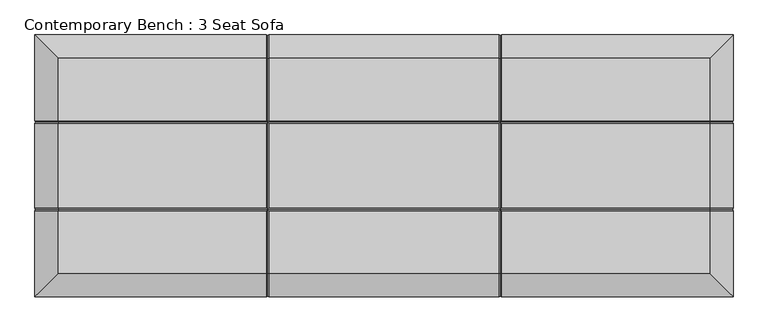
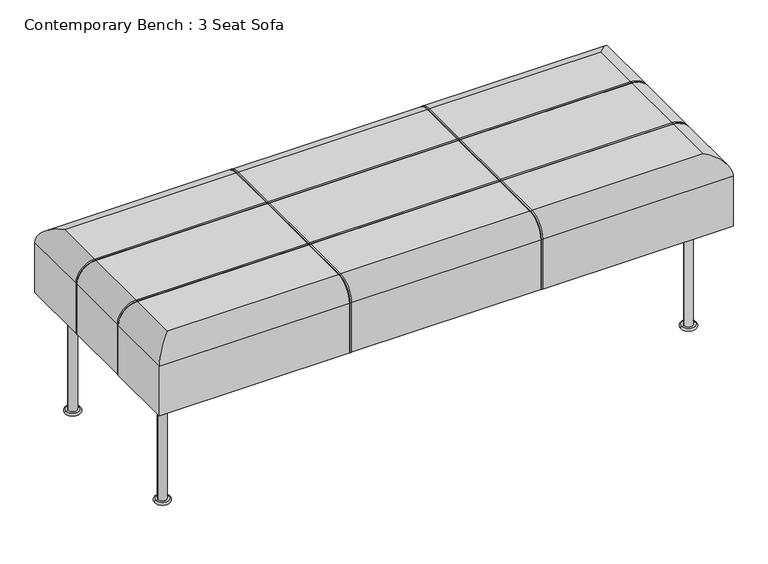
"""IFC4 building model written with IfcOpenShell, lengths in millimetres: furniture geometry, Contemporary Bench : 3 Seat Sofa."""

from ifc_helpers import new_model, si_unit, point, frame, origin, place, context, project, spatial, circle_curve, ellipse_curve, trimmed, source, transform, mapped, element, save
from ifc_brep_helpers import plane_surface, cylinder_surface, revolved_surface, advanced_brep


def contemporary_bench_3_seat_sofa_3fe76763(model_context):
    return source(origin(), model_context, "Body", "AdvancedBrep", [
        advanced_brep(
        [(662.3811933, -50.0, 5.0), (680.3811933, -50.0, 5.0), (680.3811933, -50.0, 250.0), (662.3811933, -50.0, 250.0), (657.3811933, -50.0, 5.0), (685.3811933, -50.0, 5.0), (657.3811933, -50.0, 0.0), (685.3811933, -50.0, 0.0), (671.3811933, -50.0, 0.0), (671.3811933, -50.0, 250.0)],
        [
            (0, 1, circle_curve(frame((671.3811933, -50.0, 5.0), z_axis=(0.0, 0.0, 1.0), x_axis=(1.0, 0.0, 0.0)), 9.0)),
            (1, 2),
            (2, 3, circle_curve(frame((671.3811933, -50.0, 250.0), z_axis=(0.0, 0.0, -1.0), x_axis=(1.0, 0.0, 0.0)), 9.0)),
            (3, 0),
            (1, 0, circle_curve(frame((671.3811933, -50.0, 5.0), z_axis=(0.0, 0.0, 1.0), x_axis=(1.0, 0.0, 0.0)), 9.0)),
            (3, 2, circle_curve(frame((671.3811933, -50.0, 250.0), z_axis=(0.0, 0.0, -1.0), x_axis=(1.0, 0.0, 0.0)), 9.0)),
            (4, 5, circle_curve(frame((671.3811933, -50.0, 5.0), z_axis=(0.0, 0.0, 1.0), x_axis=(1.0, 0.0, 0.0)), 14.0)),
            (5, 1),
            (0, 4),
            (5, 4, circle_curve(frame((671.3811933, -50.0, 5.0), z_axis=(0.0, 0.0, 1.0), x_axis=(1.0, 0.0, 0.0)), 14.0)),
            (6, 7, circle_curve(frame((671.3811933, -50.0, 0.0), z_axis=(0.0, 0.0, 1.0), x_axis=(1.0, 0.0, 0.0)), 14.0)),
            (7, 5, circle_curve(frame((685.3811933, -50.0, 2.5), z_axis=(0.0, -1.0, 0.0), x_axis=(-1.0, 0.0, 0.0)), 2.5)),
            (4, 6, circle_curve(frame((657.3811933, -50.0, 2.5), z_axis=(0.0, -1.0, 0.0), x_axis=(1.0, 0.0, 0.0)), 2.5)),
            (7, 6, circle_curve(frame((671.3811933, -50.0, 0.0), z_axis=(0.0, 0.0, 1.0), x_axis=(1.0, 0.0, 0.0)), 14.0)),
            (8, 7),
            (6, 8),
            (2, 9),
            (9, 3),
        ],
        [
            cylinder_surface(frame((671.3811933, -50.0, -55.0), z_axis=(0.0, 0.0, -1.0), x_axis=(1.0, 0.0, 0.0)), 9.0),
            plane_surface(frame((671.3811933, -50.0, 5.0), z_axis=(0.0, 0.0, 1.0), x_axis=(1.0, 0.0, 0.0))),
            revolved_surface(trimmed(ellipse_curve(frame((685.3811933, -50.0, 2.5), z_axis=(0.0, 1.0, 0.0), x_axis=(-1.0, 0.0, 0.0)), 2.5, 2.5), [point((685.3811933, -50.0, 5.0))], [point((685.3811933, -50.0, 0.0))], True, "CARTESIAN"), (671.3811933, -50.0, -55.0), (0.0, 0.0, -1.0)),
            plane_surface(frame((671.3811933, -50.0, 0.0), z_axis=(0.0, 0.0, -1.0), x_axis=(1.0, 0.0, 0.0))),
            plane_surface(frame((671.3811933, -50.0, 250.0), z_axis=(0.0, 0.0, 1.0), x_axis=(1.0, 0.0, 0.0))),
        ],
        [
            (0, [[1, 2, 3, 4]]),
            (0, [[5, -4, 6, -2]]),
            (1, [[7, 8, -1, 9]]),
            (1, [[10, -9, -5, -8]]),
            (2, [[11, 12, -7, 13]]),
            (2, [[14, -13, -10, -12]]),
            (3, [[15, -11, 16]]),
            (3, [[-16, -14, -15]]),
            (4, [[-3, 17, 18]]),
            (4, [[-6, -18, -17]]),
        ],
    ),
        advanced_brep(
        [(-428.6188067, -50.0, 250.0), (-437.6188067, -50.0, 250.0), (-419.6188067, -50.0, 250.0), (-414.6188067, -50.0, 0.0), (-442.6188067, -50.0, 0.0), (-428.6188067, -50.0, 0.0), (-414.6188067, -50.0, 5.0), (-442.6188067, -50.0, 5.0), (-419.6188067, -50.0, 5.0), (-437.6188067, -50.0, 5.0)],
        [
            (0, 1),
            (1, 2, circle_curve(frame((-428.6188067, -50.0, 250.0), z_axis=(0.0, 0.0, 1.0), x_axis=(-1.0, 0.0, 0.0)), 9.0)),
            (2, 0),
            (2, 1, circle_curve(frame((-428.6188067, -50.0, 250.0), z_axis=(0.0, 0.0, 1.0), x_axis=(-1.0, 0.0, 0.0)), 9.0)),
            (3, 4, circle_curve(frame((-428.6188067, -50.0, 0.0), z_axis=(0.0, 0.0, -1.0), x_axis=(-1.0, 0.0, 0.0)), 14.0)),
            (4, 5),
            (5, 3),
            (4, 3, circle_curve(frame((-428.6188067, -50.0, 0.0), z_axis=(0.0, 0.0, -1.0), x_axis=(-1.0, 0.0, 0.0)), 14.0)),
            (6, 7, circle_curve(frame((-428.6188067, -50.0, 5.0), z_axis=(0.0, 0.0, -1.0), x_axis=(-1.0, 0.0, 0.0)), 14.0)),
            (7, 4, circle_curve(frame((-442.6188067, -50.0, 2.5), z_axis=(0.0, -1.0, 0.0), x_axis=(-1.0, 0.0, 0.0)), 2.5)),
            (3, 6, circle_curve(frame((-414.6188067, -50.0, 2.5), z_axis=(0.0, -1.0, 0.0), x_axis=(1.0, 0.0, 0.0)), 2.5)),
            (7, 6, circle_curve(frame((-428.6188067, -50.0, 5.0), z_axis=(0.0, 0.0, -1.0), x_axis=(-1.0, 0.0, 0.0)), 14.0)),
            (8, 9, circle_curve(frame((-428.6188067, -50.0, 5.0), z_axis=(0.0, 0.0, -1.0), x_axis=(-1.0, 0.0, 0.0)), 9.0)),
            (9, 7),
            (6, 8),
            (9, 8, circle_curve(frame((-428.6188067, -50.0, 5.0), z_axis=(0.0, 0.0, -1.0), x_axis=(-1.0, 0.0, 0.0)), 9.0)),
            (1, 9),
            (8, 2),
        ],
        [
            plane_surface(frame((-428.6188067, -50.0, 250.0), z_axis=(0.0, 0.0, 1.0), x_axis=(-1.0, 0.0, 0.0))),
            plane_surface(frame((-428.6188067, -50.0, 0.0), z_axis=(0.0, 0.0, -1.0), x_axis=(-1.0, 0.0, 0.0))),
            revolved_surface(trimmed(ellipse_curve(frame((-442.6188067, -50.0, 2.5), z_axis=(0.0, 1.0, 0.0), x_axis=(-1.0, 0.0, 0.0)), 2.5, 2.5), [point((-442.6188067, -50.0, 0.0))], [point((-442.6188067, -50.0, 5.0))], True, "CARTESIAN"), (-428.6188067, -50.0, -55.0), (0.0, 0.0, 1.0)),
            plane_surface(frame((-428.6188067, -50.0, 5.0), z_axis=(0.0, 0.0, 1.0), x_axis=(-1.0, 0.0, 0.0))),
            cylinder_surface(frame((-428.6188067, -50.0, -55.0), z_axis=(0.0, 0.0, 1.0), x_axis=(-1.0, 0.0, 0.0)), 9.0),
        ],
        [
            (0, [[1, 2, 3]]),
            (0, [[-3, 4, -1]]),
            (1, [[5, 6, 7]]),
            (1, [[8, -7, -6]]),
            (2, [[9, 10, -5, 11]]),
            (2, [[12, -11, -8, -10]]),
            (3, [[13, 14, -9, 15]]),
            (3, [[16, -15, -12, -14]]),
            (4, [[-2, 17, -13, 18]]),
            (4, [[-4, -18, -16, -17]]),
        ],
    ),
        advanced_brep(
        [(662.3811933, -375.0, 5.0), (680.3811933, -375.0, 5.0), (680.3811933, -375.0, 250.0), (662.3811933, -375.0, 250.0), (657.3811933, -375.0, 5.0), (685.3811933, -375.0, 5.0), (657.3811933, -375.0, 0.0), (685.3811933, -375.0, 0.0), (671.3811933, -375.0, 0.0), (671.3811933, -375.0, 250.0)],
        [
            (0, 1, circle_curve(frame((671.3811933, -375.0, 5.0), z_axis=(0.0, 0.0, 1.0), x_axis=(0.9999999999999999, 0.0, 0.0)), 9.0)),
            (1, 2),
            (2, 3, circle_curve(frame((671.3811933, -375.0, 250.0), z_axis=(0.0, 0.0, -1.0), x_axis=(0.9999999999999999, 0.0, 0.0)), 9.0)),
            (3, 0),
            (1, 0, circle_curve(frame((671.3811933, -375.0, 5.0), z_axis=(0.0, 0.0, 1.0), x_axis=(0.9999999999999999, 0.0, 0.0)), 9.0)),
            (3, 2, circle_curve(frame((671.3811933, -375.0, 250.0), z_axis=(0.0, 0.0, -1.0), x_axis=(0.9999999999999999, 0.0, 0.0)), 9.0)),
            (4, 5, circle_curve(frame((671.3811933, -375.0, 5.0), z_axis=(0.0, 0.0, 1.0), x_axis=(0.9999999999999999, 0.0, 0.0)), 14.0)),
            (5, 1),
            (0, 4),
            (5, 4, circle_curve(frame((671.3811933, -375.0, 5.0), z_axis=(0.0, 0.0, 1.0), x_axis=(0.9999999999999999, 0.0, 0.0)), 14.0)),
            (6, 7, circle_curve(frame((671.3811933, -375.0, 0.0), z_axis=(0.0, 0.0, 1.0), x_axis=(0.9999999999999999, 0.0, 0.0)), 14.0)),
            (7, 5, circle_curve(frame((685.3811933, -375.0, 2.5), z_axis=(0.0, -1.0, 0.0), x_axis=(0.9999999999999999, 0.0, 0.0)), 2.5)),
            (4, 6, circle_curve(frame((657.3811933, -375.0, 2.5), z_axis=(0.0, -1.0, 0.0), x_axis=(-0.9999999999999999, 0.0, 0.0)), 2.5)),
            (7, 6, circle_curve(frame((671.3811933, -375.0, 0.0), z_axis=(0.0, 0.0, 1.0), x_axis=(0.9999999999999999, 0.0, 0.0)), 14.0)),
            (8, 7),
            (6, 8),
            (2, 9),
            (9, 3),
        ],
        [
            cylinder_surface(frame((671.3811933, -375.0, -55.0), z_axis=(0.0, 0.0, -0.9999999999999999), x_axis=(0.9999999999999999, 0.0, 0.0)), 9.0),
            plane_surface(frame((671.3811933, -375.0, 5.0), z_axis=(0.0, 0.0, 1.0), x_axis=(1.0, 0.0, 0.0))),
            revolved_surface(trimmed(ellipse_curve(frame((685.3811933, -375.0, 2.5), z_axis=(0.0, 1.0, 0.0), x_axis=(0.9999999999999999, 0.0, 0.0)), 2.5, 2.5), [point((685.3811933, -375.0, 5.0))], [point((685.3811933, -375.0, 0.0))], True, "CARTESIAN"), (671.3811933, -375.0, -55.0), (0.0, 0.0, -0.9999999999999999)),
            plane_surface(frame((671.3811933, -375.0, 0.0), z_axis=(0.0, 0.0, -1.0), x_axis=(1.0, 0.0, 0.0))),
            plane_surface(frame((671.3811933, -375.0, 250.0), z_axis=(0.0, 0.0, 1.0), x_axis=(1.0, 0.0, 0.0))),
        ],
        [
            (0, [[1, 2, 3, 4]]),
            (0, [[5, -4, 6, -2]]),
            (1, [[7, 8, -1, 9]]),
            (1, [[10, -9, -5, -8]]),
            (2, [[11, 12, -7, 13]]),
            (2, [[14, -13, -10, -12]]),
            (3, [[15, -11, 16]]),
            (3, [[-16, -14, -15]]),
            (4, [[-3, 17, 18]]),
            (4, [[-6, -18, -17]]),
        ],
    ),
        advanced_brep(
        [(-428.6188067, -375.0, 250.0), (-437.6188067, -375.0, 250.0), (-419.6188067, -375.0, 250.0), (-414.6188067, -375.0, 0.0), (-442.6188067, -375.0, 0.0), (-428.6188067, -375.0, 0.0), (-414.6188067, -375.0, 5.0), (-442.6188067, -375.0, 5.0), (-419.6188067, -375.0, 5.0), (-437.6188067, -375.0, 5.0)],
        [
            (0, 1),
            (1, 2, circle_curve(frame((-428.6188067, -375.0, 250.0), z_axis=(0.0, 0.0, 1.0), x_axis=(-1.0, 0.0, 0.0)), 9.0)),
            (2, 0),
            (2, 1, circle_curve(frame((-428.6188067, -375.0, 250.0), z_axis=(0.0, 0.0, 1.0), x_axis=(-1.0, 0.0, 0.0)), 9.0)),
            (3, 4, circle_curve(frame((-428.6188067, -375.0, 0.0), z_axis=(0.0, 0.0, -1.0), x_axis=(-1.0, 0.0, 0.0)), 14.0)),
            (4, 5),
            (5, 3),
            (4, 3, circle_curve(frame((-428.6188067, -375.0, 0.0), z_axis=(0.0, 0.0, -1.0), x_axis=(-1.0, 0.0, 0.0)), 14.0)),
            (6, 7, circle_curve(frame((-428.6188067, -375.0, 5.0), z_axis=(0.0, 0.0, -1.0), x_axis=(-1.0, 0.0, 0.0)), 14.0)),
            (7, 4, circle_curve(frame((-442.6188067, -375.0, 2.5), z_axis=(0.0, -1.0, 0.0), x_axis=(-1.0, 0.0, 0.0)), 2.5)),
            (3, 6, circle_curve(frame((-414.6188067, -375.0, 2.5), z_axis=(0.0, -1.0, 0.0), x_axis=(1.0, 0.0, 0.0)), 2.5)),
            (7, 6, circle_curve(frame((-428.6188067, -375.0, 5.0), z_axis=(0.0, 0.0, -1.0), x_axis=(-1.0, 0.0, 0.0)), 14.0)),
            (8, 9, circle_curve(frame((-428.6188067, -375.0, 5.0), z_axis=(0.0, 0.0, -1.0), x_axis=(-1.0, 0.0, 0.0)), 9.0)),
            (9, 7),
            (6, 8),
            (9, 8, circle_curve(frame((-428.6188067, -375.0, 5.0), z_axis=(0.0, 0.0, -1.0), x_axis=(-1.0, 0.0, 0.0)), 9.0)),
            (1, 9),
            (8, 2),
        ],
        [
            plane_surface(frame((-428.6188067, -375.0, 250.0), z_axis=(0.0, 0.0, 1.0), x_axis=(-1.0, 0.0, 0.0))),
            plane_surface(frame((-428.6188067, -375.0, 0.0), z_axis=(0.0, 0.0, -1.0), x_axis=(-1.0, 0.0, 0.0))),
            revolved_surface(trimmed(ellipse_curve(frame((-442.6188067, -375.0, 2.5), z_axis=(0.0, 1.0, 0.0), x_axis=(-1.0, 0.0, 0.0)), 2.5, 2.5), [point((-442.6188067, -375.0, 0.0))], [point((-442.6188067, -375.0, 5.0))], True, "CARTESIAN"), (-428.6188067, -375.0, -55.0), (0.0, 0.0, 1.0)),
            plane_surface(frame((-428.6188067, -375.0, 5.0), z_axis=(0.0, 0.0, 1.0), x_axis=(-1.0, 0.0, 0.0))),
            cylinder_surface(frame((-428.6188067, -375.0, -55.0), z_axis=(0.0, 0.0, 1.0), x_axis=(-1.0, 0.0, 0.0)), 9.0),
        ],
        [
            (0, [[1, 2, 3]]),
            (0, [[-3, 4, -1]]),
            (1, [[5, 6, 7]]),
            (1, [[8, -7, -6]]),
            (2, [[9, 10, -5, 11]]),
            (2, [[12, -11, -8, -10]]),
            (3, [[13, 14, -9, 15]]),
            (3, [[16, -15, -12, -14]]),
            (4, [[-2, 17, -13, 18]]),
            (4, [[-4, -18, -16, -17]]),
        ],
    ),
        advanced_brep(
        [(-478.6188067, -450.0, 360.0), (-478.6188067, -450.0, 250.0), (-81.2982159, -450.0, 250.0), (-81.2982159, -450.0, 360.0), (721.3811933, -450.0, 250.0), (721.3811933, -450.0, 360.0), (324.0606025, -450.0, 360.0), (324.0606025, -450.0, 250.0), (-75.9393975, -450.0, 250.0), (318.7017841, -450.0, 250.0), (318.7017841, -450.0, 360.0), (-75.9393975, -450.0, 360.0), (721.3811933, 0.0, 360.0), (721.3811933, 0.0, 250.0), (324.0606025, 0.0, 250.0), (324.0606025, 0.0, 360.0), (-478.6188067, 0.0, 250.0), (-478.6188067, 0.0, 360.0), (-81.2982159, 0.0, 360.0), (-81.2982159, 0.0, 250.0), (318.7017841, 0.0, 250.0), (-75.9393975, 0.0, 250.0), (-75.9393975, 0.0, 360.0), (318.7017841, 0.0, 360.0), (-438.6188067, -302.679408, 400.0), (-438.6188067, -410.0, 400.0), (-81.2982159, -410.0, 400.0), (-81.2982159, -302.6794092, 400.0), (-438.6188067, -40.0, 400.0), (-438.6188067, -147.3205908, 400.0), (-81.2982159, -147.3205908, 400.0), (-81.2982159, -40.0, 400.0), (-438.6188067, -152.6794084, 400.0), (-438.6188067, -297.3205908, 400.0), (-81.2982159, -297.3205908, 400.0), (-81.2982159, -152.6794092, 400.0), (681.3811933, -410.0, 400.0), (681.3811933, -302.6794092, 400.0), (324.0606025, -302.6794092, 400.0), (324.0606025, -410.0, 400.0), (681.3811933, -147.3205908, 400.0), (681.3811933, -40.0, 400.0), (324.0606025, -40.0, 400.0), (324.0606025, -147.3205908, 400.0), (681.3811933, -297.3205908, 400.0), (681.3811933, -152.6794092, 400.0), (324.0606025, -152.6794092, 400.0), (324.0606025, -297.3205908, 400.0), (318.7017854, -40.0, 400.0), (-75.9393975, -40.0, 400.0), (-75.9393975, -147.3205908, 400.0), (318.7017841, -147.3205908, 400.0), (-75.9393975, -410.0, 400.0), (318.7017841, -410.0, 400.0), (318.7017841, -302.6794092, 400.0), (-75.9393975, -302.6794092, 400.0), (-75.9393975, -297.3205908, 400.0), (318.7017841, -297.3205908, 400.0), (318.7017841, -152.6794092, 400.0), (-75.9393975, -152.6794092, 400.0), (-478.6188067, -302.6794092, 360.0), (-478.6188067, -302.6794092, 250.0), (-478.6188067, -147.3205908, 250.0), (-478.6188067, -147.3205908, 360.0), (-478.6188067, -297.3205908, 360.0), (-478.6188067, -152.6794092, 360.0), (-478.6188067, -152.6794092, 250.0), (-478.6188067, -297.3205908, 250.0), (-475.9393975, -300.0, 250.0), (-475.9393975, -150.0, 250.0), (-78.6188067, -2.6794092, 250.0), (321.3811933, -2.6794092, 250.0), (721.3811933, -147.3205908, 250.0), (718.7017841, -150.0, 250.0), (721.3811933, -152.6794092, 250.0), (721.3811933, -297.3205908, 250.0), (718.7017841, -300.0, 250.0), (721.3811933, -302.6794092, 250.0), (321.3811933, -447.3205908, 250.0), (-78.6188067, -447.3205908, 250.0), (721.3811933, -302.6794092, 360.0), (721.3811933, -147.3205908, 360.0), (721.3811933, -152.6794092, 360.0), (721.3811933, -297.3205908, 360.0), (-475.9393975, -300.0, 360.0), (-475.9393975, -150.0, 360.0), (-438.6188067, -300.0, 397.3205908), (-438.6188067, -150.0, 397.3205908), (-78.6188067, -300.0, 397.3205908), (321.3811933, -300.0, 397.3205908), (681.3811933, -300.0, 397.3205908), (-78.6188067, -150.0, 397.3205908), (321.3811933, -150.0, 397.3205908), (681.3811933, -150.0, 397.3205908), (718.7017841, -300.0, 360.0), (718.7017841, -150.0, 360.0), (-78.6188067, -2.6794092, 360.0), (321.3811933, -2.6794092, 360.0), (-78.6188067, -40.0, 397.3205908), (321.3811933, -40.0, 397.3205908), (-78.6188067, -410.0, 397.3205908), (321.3811933, -410.0, 397.3205908), (-78.6188067, -447.3205908, 360.0), (321.3811933, -447.3205908, 360.0)],
        [
            (0, 1),
            (1, 2),
            (2, 3),
            (3, 0),
            (4, 5),
            (5, 6),
            (6, 7),
            (7, 4),
            (8, 9),
            (9, 10),
            (10, 11),
            (11, 8),
            (12, 13),
            (13, 14),
            (14, 15),
            (15, 12),
            (16, 17),
            (17, 18),
            (18, 19),
            (19, 16),
            (20, 21),
            (21, 22),
            (22, 23),
            (23, 20),
            (24, 25),
            (25, 26),
            (26, 27),
            (27, 24),
            (28, 29),
            (29, 30),
            (30, 31),
            (31, 28),
            (32, 33),
            (33, 34),
            (34, 35),
            (35, 32),
            (36, 37),
            (37, 38),
            (38, 39),
            (39, 36),
            (40, 41),
            (41, 42),
            (42, 43),
            (43, 40),
            (44, 45),
            (45, 46),
            (46, 47),
            (47, 44),
            (48, 49),
            (49, 50),
            (50, 51),
            (51, 48),
            (52, 53),
            (53, 54),
            (54, 55),
            (55, 52),
            (56, 57),
            (57, 58),
            (58, 59),
            (59, 56),
            (0, 60),
            (60, 61),
            (61, 1),
            (16, 62),
            (62, 63),
            (63, 17),
            (64, 65),
            (65, 66),
            (66, 67),
            (67, 64),
            (61, 68, circle_curve(frame((-475.9393975, -302.6794092, 250.0), z_axis=(0.0, 0.0, -1.0), x_axis=(1.0, 0.0, 0.0)), 2.6794092)),
            (68, 67, circle_curve(frame((-475.9393975, -297.3205908, 250.0), z_axis=(0.0, 0.0, -1.0), x_axis=(1.0, 0.0, 0.0)), 2.6794092)),
            (66, 69, circle_curve(frame((-475.9393975, -152.6794092, 250.0), z_axis=(0.0, 0.0, -1.0), x_axis=(1.0, 0.0, 0.0)), 2.6794092)),
            (69, 62, circle_curve(frame((-475.9393975, -147.3205908, 250.0), z_axis=(0.0, 0.0, -1.0), x_axis=(1.0, 0.0, 0.0)), 2.6794092)),
            (19, 70, circle_curve(frame((-81.2982159, -2.6794092, 250.0), z_axis=(0.0, 0.0, -1.0), x_axis=(1.0, 0.0, 0.0)), 2.6794092)),
            (70, 21, circle_curve(frame((-75.9393975, -2.6794092, 250.0), z_axis=(0.0, 0.0, -1.0), x_axis=(1.0, 0.0, 0.0)), 2.6794092)),
            (20, 71, circle_curve(frame((318.7017841, -2.6794092, 250.0), z_axis=(0.0, 0.0, -1.0), x_axis=(1.0, 0.0, 0.0)), 2.6794092)),
            (71, 14, circle_curve(frame((324.0606025, -2.6794092, 250.0), z_axis=(0.0, 0.0, -1.0), x_axis=(1.0, 0.0, 0.0)), 2.6794092)),
            (13, 72),
            (72, 73, circle_curve(frame((718.7017841, -147.3205908, 250.0), z_axis=(0.0, 0.0, -1.0), x_axis=(-1.0, 0.0, 0.0)), 2.6794092)),
            (73, 74, circle_curve(frame((718.7017841, -152.6794092, 250.0), z_axis=(0.0, 0.0, -1.0), x_axis=(-1.0, 0.0, 0.0)), 2.6794092)),
            (74, 75),
            (75, 76, circle_curve(frame((718.7017841, -297.3205908, 250.0), z_axis=(0.0, 0.0, -1.0), x_axis=(-1.0, 0.0, 0.0)), 2.6794092)),
            (76, 77, circle_curve(frame((718.7017841, -302.6794092, 250.0), z_axis=(0.0, 0.0, -1.0), x_axis=(-1.0, 0.0, 0.0)), 2.6794092)),
            (77, 4),
            (7, 78, circle_curve(frame((324.0606025, -447.3205908, 250.0), z_axis=(0.0, 0.0, -1.0), x_axis=(1.0, 0.0, 0.0)), 2.6794092)),
            (78, 9, circle_curve(frame((318.7017841, -447.3205908, 250.0), z_axis=(0.0, 0.0, -1.0), x_axis=(1.0, 0.0, 0.0)), 2.6794092)),
            (8, 79, circle_curve(frame((-75.9393975, -447.3205908, 250.0), z_axis=(0.0, 0.0, -1.0), x_axis=(1.0, 0.0, 0.0)), 2.6794092)),
            (79, 2, circle_curve(frame((-81.2982159, -447.3205908, 250.0), z_axis=(0.0, 0.0, -1.0), x_axis=(1.0, 0.0, 0.0)), 2.6794092)),
            (77, 80),
            (80, 5),
            (12, 81),
            (81, 72),
            (74, 82),
            (82, 83),
            (83, 75),
            (32, 65, circle_curve(frame((-438.6188067, -152.6794092, 360.0), z_axis=(0.0, -1.0, 0.0), x_axis=(-1.0, 0.0, 0.0)), 40.0)),
            (64, 33, circle_curve(frame((-438.6188067, -297.3205908, 360.0), z_axis=(0.0, 1.0, 0.0), x_axis=(-1.0, 0.0, 0.0)), 40.0)),
            (28, 17, ellipse_curve(frame((-438.6188067, -40.0, 360.0), z_axis=(-0.7071067811865475, -0.7071067811865475, 0.0), x_axis=(-0.7071067811865474, 0.7071067811865476, 0.0)), 56.5685425, 40.0)),
            (63, 29, circle_curve(frame((-438.6188067, -147.3205908, 360.0), z_axis=(0.0, 1.0, 0.0), x_axis=(-1.0, 0.0, 0.0)), 40.0)),
            (0, 25, ellipse_curve(frame((-438.6188067, -410.0, 360.0), z_axis=(-0.7071067811865475, 0.7071067811865475, 0.0), x_axis=(0.7071067811865474, 0.7071067811865476, 0.0)), 56.5685425, 40.0)),
            (24, 60, circle_curve(frame((-438.6188067, -302.6794092, 360.0), z_axis=(0.0, -1.0, 0.0), x_axis=(-1.0, 0.0, 0.0)), 40.0)),
            (22, 49, circle_curve(frame((-75.9393975, -40.0, 360.0), z_axis=(1.0, 0.0, 0.0), x_axis=(0.0, 1.0, 0.0)), 40.0)),
            (48, 23, circle_curve(frame((318.7017841, -40.0, 360.0), z_axis=(-1.0, 0.0, 0.0), x_axis=(0.0, 1.0, 0.0)), 40.0)),
            (31, 18, circle_curve(frame((-81.2982159, -40.0, 360.0), z_axis=(-1.0, 0.0, 0.0), x_axis=(0.0, 1.0, 0.0)), 40.0)),
            (41, 12, ellipse_curve(frame((681.3811933, -40.0, 360.0), z_axis=(-0.7071067811865475, 0.7071067811865475, 0.0), x_axis=(0.7071067811865476, 0.7071067811865474, 0.0)), 56.5685425, 40.0)),
            (15, 42, circle_curve(frame((324.0606025, -40.0, 360.0), z_axis=(1.0, 0.0, 0.0), x_axis=(0.0, 1.0, 0.0)), 40.0)),
            (44, 83, circle_curve(frame((681.3811933, -297.3205908, 360.0), z_axis=(0.0, 1.0, 0.0), x_axis=(1.0, 0.0, 0.0)), 40.0)),
            (82, 45, circle_curve(frame((681.3811933, -152.6794092, 360.0), z_axis=(0.0, -1.0, 0.0), x_axis=(1.0, 0.0, 0.0)), 40.0)),
            (40, 81, circle_curve(frame((681.3811933, -147.3205908, 360.0), z_axis=(0.0, 1.0, 0.0), x_axis=(1.0, 0.0, 0.0)), 40.0)),
            (36, 5, ellipse_curve(frame((681.3811933, -410.0, 360.0), z_axis=(0.7071067811865475, 0.7071067811865475, 0.0), x_axis=(0.7071067811865474, -0.7071067811865476, 0.0)), 56.5685425, 40.0)),
            (80, 37, circle_curve(frame((681.3811933, -302.6794092, 360.0), z_axis=(0.0, -1.0, 0.0), x_axis=(1.0, 0.0, 0.0)), 40.0)),
            (10, 53, circle_curve(frame((318.7017841, -410.0, 360.0), z_axis=(-1.0, 0.0, 0.0), x_axis=(0.0, -1.0, 0.0)), 40.0)),
            (52, 11, circle_curve(frame((-75.9393975, -410.0, 360.0), z_axis=(1.0, 0.0, 0.0), x_axis=(0.0, -1.0, 0.0)), 40.0)),
            (3, 26, circle_curve(frame((-81.2982159, -410.0, 360.0), z_axis=(-1.0, 0.0, 0.0), x_axis=(0.0, -1.0, 0.0)), 40.0)),
            (39, 6, circle_curve(frame((324.0606025, -410.0, 360.0), z_axis=(1.0, 0.0, 0.0), x_axis=(0.0, -1.0, 0.0)), 40.0)),
            (68, 84),
            (84, 64, circle_curve(frame((-475.9393975, -297.3205908, 360.0), z_axis=(0.0, 0.0, -1.0), x_axis=(1.0, 0.0, 0.0)), 2.6794092)),
            (60, 84, circle_curve(frame((-475.9393975, -302.6794092, 360.0), z_axis=(0.0, 0.0, -1.0), x_axis=(1.0, 0.0, 0.0)), 2.6794092)),
            (69, 85),
            (85, 63, circle_curve(frame((-475.9393975, -147.3205908, 360.0), z_axis=(0.0, 0.0, -1.0), x_axis=(1.0, 0.0, 0.0)), 2.6794092)),
            (65, 85, circle_curve(frame((-475.9393975, -152.6794092, 360.0), z_axis=(0.0, 0.0, -1.0), x_axis=(1.0, 0.0, 0.0)), 2.6794092)),
            (84, 86, circle_curve(frame((-438.6188067, -300.0, 360.0), z_axis=(0.0, 1.0, 0.0), x_axis=(-1.0, 0.0, 0.0)), 37.3205908)),
            (86, 33, circle_curve(frame((-438.6188067, -297.3205908, 397.3205908), z_axis=(-1.0, 0.0, 0.0), x_axis=(0.0, 0.0, -1.0)), 2.6794092)),
            (24, 86, circle_curve(frame((-438.6188067, -302.6794092, 397.3205908), z_axis=(-1.0, 0.0, 0.0), x_axis=(0.0, 0.0, -1.0)), 2.6794092)),
            (85, 87, circle_curve(frame((-438.6188067, -150.0, 360.0), z_axis=(0.0, 1.0, 0.0), x_axis=(-1.0, 0.0, 0.0)), 37.3205908)),
            (87, 29, circle_curve(frame((-438.6188067, -147.3205908, 397.3205908), z_axis=(-1.0, 0.0, 0.0), x_axis=(0.0, 0.0, -1.0)), 2.6794092)),
            (32, 87, circle_curve(frame((-438.6188067, -152.6794092, 397.3205908), z_axis=(-1.0, 0.0, 0.0), x_axis=(0.0, 0.0, -1.0)), 2.6794092)),
            (56, 88, ellipse_curve(frame((-75.9393975, -297.3205908, 397.3205908), z_axis=(0.7071067811865464, -0.7071067811865487, 0.0), x_axis=(0.7071067811865487, 0.7071067811865464, 0.0)), 3.7892569, 2.6794092)),
            (88, 89),
            (89, 57, ellipse_curve(frame((318.7017841, -297.3205908, 397.3205908), z_axis=(-0.7071067811865487, -0.7071067811865464, 0.0), x_axis=(0.7071067811865465, -0.7071067811865487, 0.0)), 3.7892569, 2.6794092)),
            (86, 88),
            (88, 34, ellipse_curve(frame((-81.2982159, -297.3205908, 397.3205908), z_axis=(-0.7071067811865487, -0.7071067811865464, 0.0), x_axis=(0.7071067811865465, -0.7071067811865487, 0.0)), 3.7892569, 2.6794092)),
            (90, 44, circle_curve(frame((681.3811933, -297.3205908, 397.3205908), z_axis=(-1.0, 0.0, 0.0), x_axis=(0.0, 0.0, -1.0)), 2.6794092)),
            (47, 89, ellipse_curve(frame((324.0606025, -297.3205908, 397.3205908), z_axis=(0.7071067811865464, -0.7071067811865487, 0.0), x_axis=(0.7071067811865487, 0.7071067811865464, 0.0)), 3.7892569, 2.6794092)),
            (89, 90),
            (54, 89, ellipse_curve(frame((318.7017841, -302.6794092, 397.3205908), z_axis=(-0.7071067811865464, 0.7071067811865487, 0.0), x_axis=(0.7071067811865487, 0.7071067811865464, 0.0)), 3.7892569, 2.6794092)),
            (88, 55, ellipse_curve(frame((-75.9393975, -302.6794092, 397.3205908), z_axis=(0.7071067811865487, 0.7071067811865464, 0.0), x_axis=(0.7071067811865465, -0.7071067811865487, 0.0)), 3.7892569, 2.6794092)),
            (27, 88, ellipse_curve(frame((-81.2982159, -302.6794092, 397.3205908), z_axis=(-0.7071067811865464, 0.7071067811865487, 0.0), x_axis=(0.7071067811865487, 0.7071067811865464, 0.0)), 3.7892569, 2.6794092)),
            (37, 90, circle_curve(frame((681.3811933, -302.6794092, 397.3205908), z_axis=(-1.0, 0.0, 0.0), x_axis=(0.0, 0.0, -1.0)), 2.6794092)),
            (89, 38, ellipse_curve(frame((324.0606025, -302.6794092, 397.3205908), z_axis=(0.7071067811865487, 0.7071067811865464, 0.0), x_axis=(0.7071067811865465, -0.7071067811865487, 0.0)), 3.7892569, 2.6794092)),
            (50, 91, ellipse_curve(frame((-75.9393975, -147.3205908, 397.3205908), z_axis=(0.7071067811865464, -0.7071067811865487, 0.0), x_axis=(0.7071067811865487, 0.7071067811865464, 0.0)), 3.7892569, 2.6794092)),
            (91, 92),
            (92, 51, ellipse_curve(frame((318.7017841, -147.3205908, 397.3205908), z_axis=(-0.7071067811865487, -0.7071067811865464, 0.0), x_axis=(0.7071067811865465, -0.7071067811865487, 0.0)), 3.7892569, 2.6794092)),
            (87, 91),
            (91, 30, ellipse_curve(frame((-81.2982159, -147.3205908, 397.3205908), z_axis=(-0.7071067811865487, -0.7071067811865464, 0.0), x_axis=(0.7071067811865465, -0.7071067811865487, 0.0)), 3.7892569, 2.6794092)),
            (93, 40, circle_curve(frame((681.3811933, -147.3205908, 397.3205908), z_axis=(-1.0, 0.0, 0.0), x_axis=(0.0, 0.0, -1.0)), 2.6794092)),
            (43, 92, ellipse_curve(frame((324.0606025, -147.3205908, 397.3205908), z_axis=(0.7071067811865464, -0.7071067811865487, 0.0), x_axis=(0.7071067811865487, 0.7071067811865464, 0.0)), 3.7892569, 2.6794092)),
            (92, 93),
            (58, 92, ellipse_curve(frame((318.7017841, -152.6794092, 397.3205908), z_axis=(-0.7071067811865464, 0.7071067811865487, 0.0), x_axis=(0.7071067811865487, 0.7071067811865464, 0.0)), 3.7892569, 2.6794092)),
            (91, 59, ellipse_curve(frame((-75.9393975, -152.6794092, 397.3205908), z_axis=(0.7071067811865487, 0.7071067811865464, 0.0), x_axis=(0.7071067811865465, -0.7071067811865487, 0.0)), 3.7892569, 2.6794092)),
            (35, 91, ellipse_curve(frame((-81.2982159, -152.6794092, 397.3205908), z_axis=(-0.7071067811865464, 0.7071067811865487, 0.0), x_axis=(0.7071067811865487, 0.7071067811865464, 0.0)), 3.7892569, 2.6794092)),
            (45, 93, circle_curve(frame((681.3811933, -152.6794092, 397.3205908), z_axis=(-1.0, 0.0, 0.0), x_axis=(0.0, 0.0, -1.0)), 2.6794092)),
            (92, 46, ellipse_curve(frame((324.0606025, -152.6794092, 397.3205908), z_axis=(0.7071067811865487, 0.7071067811865464, 0.0), x_axis=(0.7071067811865465, -0.7071067811865487, 0.0)), 3.7892569, 2.6794092)),
            (90, 94, circle_curve(frame((681.3811933, -300.0, 360.0), z_axis=(0.0, 1.0, 0.0), x_axis=(0.0, 0.0, 1.0)), 37.3205908)),
            (94, 83, circle_curve(frame((718.7017841, -297.3205908, 360.0), z_axis=(0.0, 0.0, 1.0), x_axis=(-1.0, 0.0, 0.0)), 2.6794092)),
            (80, 94, circle_curve(frame((718.7017841, -302.6794092, 360.0), z_axis=(0.0, 0.0, 1.0), x_axis=(-1.0, 0.0, 0.0)), 2.6794092)),
            (93, 95, circle_curve(frame((681.3811933, -150.0, 360.0), z_axis=(0.0, 1.0, 0.0), x_axis=(0.0, 0.0, 1.0)), 37.3205908)),
            (95, 81, circle_curve(frame((718.7017841, -147.3205908, 360.0), z_axis=(0.0, 0.0, 1.0), x_axis=(-1.0, 0.0, 0.0)), 2.6794092)),
            (82, 95, circle_curve(frame((718.7017841, -152.6794092, 360.0), z_axis=(0.0, 0.0, 1.0), x_axis=(-1.0, 0.0, 0.0)), 2.6794092)),
            (94, 76),
            (95, 73),
            (70, 96),
            (96, 22, circle_curve(frame((-75.9393975, -2.6794092, 360.0), z_axis=(0.0, 0.0, -1.0), x_axis=(1.0, 0.0, 0.0)), 2.6794092)),
            (18, 96, circle_curve(frame((-81.2982159, -2.6794092, 360.0), z_axis=(0.0, 0.0, -1.0), x_axis=(1.0, 0.0, 0.0)), 2.6794092)),
            (71, 97),
            (97, 15, circle_curve(frame((324.0606025, -2.6794092, 360.0), z_axis=(0.0, 0.0, -1.0), x_axis=(1.0, 0.0, 0.0)), 2.6794092)),
            (23, 97, circle_curve(frame((318.7017841, -2.6794092, 360.0), z_axis=(0.0, 0.0, -1.0), x_axis=(1.0, 0.0, 0.0)), 2.6794092)),
            (96, 98, circle_curve(frame((-78.6188067, -40.0, 360.0), z_axis=(1.0, 0.0, 0.0), x_axis=(0.0, 1.0, 0.0)), 37.3205908)),
            (98, 49, circle_curve(frame((-75.9393975, -40.0, 397.3205908), z_axis=(0.0, 1.0, 0.0), x_axis=(1.0, 0.0, 0.0)), 2.6794092)),
            (31, 98, circle_curve(frame((-81.2982159, -40.0, 397.3205908), z_axis=(0.0, 1.0, 0.0), x_axis=(1.0, 0.0, 0.0)), 2.6794092)),
            (97, 99, circle_curve(frame((321.3811933, -40.0, 360.0), z_axis=(1.0, 0.0, 0.0), x_axis=(0.0, 1.0, 0.0)), 37.3205908)),
            (99, 42, circle_curve(frame((324.0606025, -40.0, 397.3205908), z_axis=(0.0, 1.0, 0.0), x_axis=(1.0, 0.0, 0.0)), 2.6794092)),
            (48, 99, circle_curve(frame((318.7017841, -40.0, 397.3205908), z_axis=(0.0, 1.0, 0.0), x_axis=(1.0, 0.0, 0.0)), 2.6794092)),
            (98, 91),
            (100, 52, circle_curve(frame((-75.9393975, -410.0, 397.3205908), z_axis=(0.0, 1.0, 0.0), x_axis=(1.0, 0.0, 0.0)), 2.6794092)),
            (88, 100),
            (91, 88),
            (26, 100, circle_curve(frame((-81.2982159, -410.0, 397.3205908), z_axis=(0.0, 1.0, 0.0), x_axis=(1.0, 0.0, 0.0)), 2.6794092)),
            (99, 92),
            (101, 39, circle_curve(frame((324.0606025, -410.0, 397.3205908), z_axis=(0.0, 1.0, 0.0), x_axis=(1.0, 0.0, 0.0)), 2.6794092)),
            (89, 101),
            (92, 89),
            (53, 101, circle_curve(frame((318.7017841, -410.0, 397.3205908), z_axis=(0.0, 1.0, 0.0), x_axis=(1.0, 0.0, 0.0)), 2.6794092)),
            (100, 102, circle_curve(frame((-78.6188067, -410.0, 360.0), z_axis=(1.0, 0.0, 0.0), x_axis=(0.0, 0.0, 1.0)), 37.3205908)),
            (102, 11, circle_curve(frame((-75.9393975, -447.3205908, 360.0), z_axis=(0.0, 0.0, 1.0), x_axis=(1.0, 0.0, 0.0)), 2.6794092)),
            (3, 102, circle_curve(frame((-81.2982159, -447.3205908, 360.0), z_axis=(0.0, 0.0, 1.0), x_axis=(1.0, 0.0, 0.0)), 2.6794092)),
            (101, 103, circle_curve(frame((321.3811933, -410.0, 360.0), z_axis=(1.0, 0.0, 0.0), x_axis=(0.0, 0.0, 1.0)), 37.3205908)),
            (103, 6, circle_curve(frame((324.0606025, -447.3205908, 360.0), z_axis=(0.0, 0.0, 1.0), x_axis=(1.0, 0.0, 0.0)), 2.6794092)),
            (10, 103, circle_curve(frame((318.7017841, -447.3205908, 360.0), z_axis=(0.0, 0.0, 1.0), x_axis=(1.0, 0.0, 0.0)), 2.6794092)),
            (102, 79),
            (103, 78),
        ],
        [
            plane_surface(frame((-478.6188067, -450.0, 400.0), z_axis=(0.0, -1.0, 0.0), x_axis=(-1.0, 0.0, 0.0))),
            plane_surface(frame((-478.6188067, 0.0, 400.0), z_axis=(0.0, 1.0, 0.0), x_axis=(1.0, 0.0, 0.0))),
            plane_surface(frame((721.3811933, -450.0, 400.0), z_axis=(0.0, 0.0, 1.0), x_axis=(0.0, 1.0, 0.0))),
            plane_surface(frame((-478.6188067, -450.0, 400.0), z_axis=(-1.0, 0.0, 0.0), x_axis=(0.0, 1.0, 0.0))),
            plane_surface(frame((-478.6188067, -450.0, 250.0), z_axis=(0.0, 0.0, -1.0), x_axis=(0.0, 1.0, 0.0))),
            plane_surface(frame((721.3811933, -450.0, 250.0), z_axis=(1.0, 0.0, 0.0), x_axis=(0.0, 1.0, 0.0))),
            cylinder_surface(frame((-438.6188067, -450.0, 360.0), z_axis=(0.0, 1.0, 0.0), x_axis=(-1.0, 0.0, 0.0)), 40.0),
            cylinder_surface(frame((-478.6188067, -40.0, 360.0), z_axis=(1.0, 0.0, 0.0), x_axis=(0.0, 1.0, 0.0)), 40.0),
            cylinder_surface(frame((681.3811933, 0.0, 360.0), z_axis=(0.0, -1.0, 0.0), x_axis=(1.0, 0.0, 0.0)), 40.0),
            cylinder_surface(frame((721.3811933, -410.0, 360.0), z_axis=(-1.0, 0.0, 0.0), x_axis=(0.0, -1.0, 0.0)), 40.0),
            cylinder_surface(frame((-475.9393975, -297.3205908, 250.0), z_axis=(0.0, 0.0, 1.0), x_axis=(1.0, 0.0, 0.0)), 2.6794092),
            cylinder_surface(frame((-475.9393975, -302.6794092, 250.0), z_axis=(0.0, 0.0, 1.0), x_axis=(1.0, 0.0, 0.0)), 2.6794092),
            cylinder_surface(frame((-475.9393975, -147.3205908, 250.0), z_axis=(0.0, 0.0, 1.0), x_axis=(1.0, 0.0, 0.0)), 2.6794092),
            cylinder_surface(frame((-475.9393975, -152.6794092, 250.0), z_axis=(0.0, 0.0, 1.0), x_axis=(1.0, 0.0, 0.0)), 2.6794092),
            revolved_surface(trimmed(ellipse_curve(frame((-475.9393975, -297.3205908, 360.0), z_axis=(0.0, 0.0, -1.0), x_axis=(1.0, 0.0, 0.0)), 2.6794092, 2.6794092), [point((-475.9393975, -300.0, 360.0))], [point((-478.6188067, -297.3205908, 360.0))], True, "CARTESIAN"), (-438.6188067, -375.0, 360.0), (0.0, 1.0, 0.0)),
            revolved_surface(trimmed(ellipse_curve(frame((-475.9393975, -302.6794092, 360.0), z_axis=(0.0, 0.0, -1.0), x_axis=(1.0, 0.0, 0.0)), 2.6794092, 2.6794092), [point((-478.6188067, -302.6794092, 360.0))], [point((-475.9393975, -300.0, 360.0))], True, "CARTESIAN"), (-438.6188067, -375.0, 360.0), (0.0, 1.0, 0.0)),
            revolved_surface(trimmed(ellipse_curve(frame((-475.9393975, -147.3205908, 360.0), z_axis=(0.0, 0.0, -1.0), x_axis=(1.0, 0.0, 0.0)), 2.6794092, 2.6794092), [point((-475.9393975, -150.0, 360.0))], [point((-478.6188067, -147.3205908, 360.0))], True, "CARTESIAN"), (-438.6188067, -375.0, 360.0), (0.0, 1.0, 0.0)),
            revolved_surface(trimmed(ellipse_curve(frame((-475.9393975, -152.6794092, 360.0), z_axis=(0.0, 0.0, -1.0), x_axis=(1.0, 0.0, 0.0)), 2.6794092, 2.6794092), [point((-478.6188067, -152.6794092, 360.0))], [point((-475.9393975, -150.0, 360.0))], True, "CARTESIAN"), (-438.6188067, -375.0, 360.0), (0.0, 1.0, 0.0)),
            cylinder_surface(frame((-438.6188067, -297.3205908, 397.3205908), z_axis=(1.0, 0.0, 0.0), x_axis=(0.0, 0.0, -1.0)), 2.6794092),
            cylinder_surface(frame((-438.6188067, -302.6794092, 397.3205908), z_axis=(1.0, 0.0, 0.0), x_axis=(0.0, 0.0, -1.0)), 2.6794092),
            cylinder_surface(frame((-438.6188067, -147.3205908, 397.3205908), z_axis=(1.0, 0.0, 0.0), x_axis=(0.0, 0.0, -1.0)), 2.6794092),
            cylinder_surface(frame((-438.6188067, -152.6794092, 397.3205908), z_axis=(1.0, 0.0, 0.0), x_axis=(0.0, 0.0, -1.0)), 2.6794092),
            revolved_surface(trimmed(ellipse_curve(frame((681.3811933, -297.3205908, 397.3205908), z_axis=(-1.0, 0.0, 0.0), x_axis=(0.0, 0.0, -1.0)), 2.6794092, 2.6794092), [point((681.3811933, -300.0, 397.3205908))], [point((681.3811933, -297.3205908, 400.0))], True, "CARTESIAN"), (681.3811933, -375.0, 360.0), (0.0, 1.0, 0.0)),
            revolved_surface(trimmed(ellipse_curve(frame((681.3811933, -302.6794092, 397.3205908), z_axis=(-1.0, 0.0, 0.0), x_axis=(0.0, 0.0, -1.0)), 2.6794092, 2.6794092), [point((681.3811933, -302.6794092, 400.0))], [point((681.3811933, -300.0, 397.3205908))], True, "CARTESIAN"), (681.3811933, -375.0, 360.0), (0.0, 1.0, 0.0)),
            revolved_surface(trimmed(ellipse_curve(frame((681.3811933, -147.3205908, 397.3205908), z_axis=(-1.0, 0.0, 0.0), x_axis=(0.0, 0.0, -1.0)), 2.6794092, 2.6794092), [point((681.3811933, -150.0, 397.3205908))], [point((681.3811933, -147.3205908, 400.0))], True, "CARTESIAN"), (681.3811933, -375.0, 360.0), (0.0, 1.0, 0.0)),
            revolved_surface(trimmed(ellipse_curve(frame((681.3811933, -152.6794092, 397.3205908), z_axis=(-1.0, 0.0, 0.0), x_axis=(0.0, 0.0, -1.0)), 2.6794092, 2.6794092), [point((681.3811933, -152.6794092, 400.0))], [point((681.3811933, -150.0, 397.3205908))], True, "CARTESIAN"), (681.3811933, -375.0, 360.0), (0.0, 1.0, 0.0)),
            cylinder_surface(frame((718.7017841, -297.3205908, 360.0), z_axis=(0.0, 0.0, -1.0), x_axis=(-1.0, 0.0, 0.0)), 2.6794092),
            cylinder_surface(frame((718.7017841, -302.6794092, 360.0), z_axis=(0.0, 0.0, -1.0), x_axis=(-1.0, 0.0, 0.0)), 2.6794092),
            cylinder_surface(frame((718.7017841, -147.3205908, 360.0), z_axis=(0.0, 0.0, -1.0), x_axis=(-1.0, 0.0, 0.0)), 2.6794092),
            cylinder_surface(frame((718.7017841, -152.6794092, 360.0), z_axis=(0.0, 0.0, -1.0), x_axis=(-1.0, 0.0, 0.0)), 2.6794092),
            cylinder_surface(frame((-75.9393975, -2.6794092, 250.0), z_axis=(0.0, 0.0, 1.0), x_axis=(1.0, 0.0, 0.0)), 2.6794092),
            cylinder_surface(frame((-81.2982159, -2.6794092, 250.0), z_axis=(0.0, 0.0, 1.0), x_axis=(1.0, 0.0, 0.0)), 2.6794092),
            cylinder_surface(frame((324.0606025, -2.6794092, 250.0), z_axis=(0.0, 0.0, 1.0), x_axis=(1.0, 0.0, 0.0)), 2.6794092),
            cylinder_surface(frame((318.7017841, -2.6794092, 250.0), z_axis=(0.0, 0.0, 1.0), x_axis=(1.0, 0.0, 0.0)), 2.6794092),
            revolved_surface(trimmed(ellipse_curve(frame((-75.9393975, -2.6794092, 360.0), z_axis=(0.0, 0.0, -1.0), x_axis=(1.0, 0.0, 0.0)), 2.6794092, 2.6794092), [point((-78.6188067, -2.6794092, 360.0))], [point((-75.9393975, 0.0, 360.0))], True, "CARTESIAN"), (121.3811933, -40.0, 360.0), (1.0, 0.0, 0.0)),
            revolved_surface(trimmed(ellipse_curve(frame((-81.2982159, -2.6794092, 360.0), z_axis=(0.0, 0.0, -1.0), x_axis=(1.0, 0.0, 0.0)), 2.6794092, 2.6794092), [point((-81.2982159, 0.0, 360.0))], [point((-78.6188067, -2.6794092, 360.0))], True, "CARTESIAN"), (121.3811933, -40.0, 360.0), (1.0, 0.0, 0.0)),
            revolved_surface(trimmed(ellipse_curve(frame((324.0606025, -2.6794092, 360.0), z_axis=(0.0, 0.0, -1.0), x_axis=(1.0, 0.0, 0.0)), 2.6794092, 2.6794092), [point((321.3811933, -2.6794092, 360.0))], [point((324.0606025, 0.0, 360.0))], True, "CARTESIAN"), (121.3811933, -40.0, 360.0), (1.0, 0.0, 0.0)),
            revolved_surface(trimmed(ellipse_curve(frame((318.7017841, -2.6794092, 360.0), z_axis=(0.0, 0.0, -1.0), x_axis=(1.0, 0.0, 0.0)), 2.6794092, 2.6794092), [point((318.7017841, 0.0, 360.0))], [point((321.3811933, -2.6794092, 360.0))], True, "CARTESIAN"), (121.3811933, -40.0, 360.0), (1.0, 0.0, 0.0)),
            cylinder_surface(frame((-75.9393975, -40.0, 397.3205908), z_axis=(0.0, -1.0, 0.0), x_axis=(1.0, 0.0, 0.0)), 2.6794092),
            cylinder_surface(frame((-81.2982159, -40.0, 397.3205908), z_axis=(0.0, -1.0, 0.0), x_axis=(1.0, 0.0, 0.0)), 2.6794092),
            cylinder_surface(frame((324.0606025, -40.0, 397.3205908), z_axis=(0.0, -1.0, 0.0), x_axis=(1.0, 0.0, 0.0)), 2.6794092),
            cylinder_surface(frame((318.7017841, -40.0, 397.3205908), z_axis=(0.0, -1.0, 0.0), x_axis=(1.0, 0.0, 0.0)), 2.6794092),
            revolved_surface(trimmed(ellipse_curve(frame((-75.9393975, -410.0, 397.3205908), z_axis=(0.0, 1.0, 0.0), x_axis=(1.0, 0.0, 0.0)), 2.6794092, 2.6794092), [point((-78.6188067, -410.0, 397.3205908))], [point((-75.9393975, -410.0, 400.0))], True, "CARTESIAN"), (121.3811933, -410.0, 360.0), (1.0, 0.0, 0.0)),
            revolved_surface(trimmed(ellipse_curve(frame((-81.2982159, -410.0, 397.3205908), z_axis=(0.0, 1.0, 0.0), x_axis=(1.0, 0.0, 0.0)), 2.6794092, 2.6794092), [point((-81.2982159, -410.0, 400.0))], [point((-78.6188067, -410.0, 397.3205908))], True, "CARTESIAN"), (121.3811933, -410.0, 360.0), (1.0, 0.0, 0.0)),
            revolved_surface(trimmed(ellipse_curve(frame((324.0606025, -410.0, 397.3205908), z_axis=(0.0, 1.0, 0.0), x_axis=(1.0, 0.0, 0.0)), 2.6794092, 2.6794092), [point((321.3811933, -410.0, 397.3205908))], [point((324.0606025, -410.0, 400.0))], True, "CARTESIAN"), (121.3811933, -410.0, 360.0), (1.0, 0.0, 0.0)),
            revolved_surface(trimmed(ellipse_curve(frame((318.7017841, -410.0, 397.3205908), z_axis=(0.0, 1.0, 0.0), x_axis=(1.0, 0.0, 0.0)), 2.6794092, 2.6794092), [point((318.7017841, -410.0, 400.0))], [point((321.3811933, -410.0, 397.3205908))], True, "CARTESIAN"), (121.3811933, -410.0, 360.0), (1.0, 0.0, 0.0)),
            cylinder_surface(frame((-75.9393975, -447.3205908, 360.0), z_axis=(0.0, 0.0, -1.0), x_axis=(1.0, 0.0, 0.0)), 2.6794092),
            cylinder_surface(frame((-81.2982159, -447.3205908, 360.0), z_axis=(0.0, 0.0, -1.0), x_axis=(1.0, 0.0, 0.0)), 2.6794092),
            cylinder_surface(frame((324.0606025, -447.3205908, 360.0), z_axis=(0.0, 0.0, -1.0), x_axis=(1.0, 0.0, 0.0)), 2.6794092),
            cylinder_surface(frame((318.7017841, -447.3205908, 360.0), z_axis=(0.0, 0.0, -1.0), x_axis=(1.0, 0.0, 0.0)), 2.6794092),
        ],
        [
            (0, [[1, 2, 3, 4]]),
            (0, [[5, 6, 7, 8]]),
            (0, [[9, 10, 11, 12]]),
            (1, [[13, 14, 15, 16]]),
            (1, [[17, 18, 19, 20]]),
            (1, [[21, 22, 23, 24]]),
            (2, [[25, 26, 27, 28]]),
            (2, [[29, 30, 31, 32]]),
            (2, [[33, 34, 35, 36]]),
            (2, [[37, 38, 39, 40]]),
            (2, [[41, 42, 43, 44]]),
            (2, [[45, 46, 47, 48]]),
            (2, [[49, 50, 51, 52]]),
            (2, [[53, 54, 55, 56]]),
            (2, [[57, 58, 59, 60]]),
            (3, [[-1, 61, 62, 63]]),
            (3, [[-17, 64, 65, 66]]),
            (3, [[67, 68, 69, 70]]),
            (4, [[-63, 71, 72, -69, 73, 74, -64, -20, 75, 76, -21, 77, 78, -14, 79, 80, 81, 82, 83, 84, 85, -8, 86, 87, -9, 88, 89, -2]]),
            (5, [[-5, -85, 90, 91]]),
            (5, [[-13, 92, 93, -79]]),
            (5, [[-82, 94, 95, 96]]),
            (6, [[-33, 97, -67, 98]]),
            (6, [[99, -66, 100, -29]]),
            (6, [[101, -25, 102, -61]]),
            (7, [[-23, 103, -49, 104]]),
            (7, [[-99, -32, 105, -18]]),
            (7, [[106, -16, 107, -42]]),
            (8, [[-45, 108, -95, 109]]),
            (8, [[-106, -41, 110, -92]]),
            (8, [[111, -91, 112, -37]]),
            (9, [[-11, 113, -53, 114]]),
            (9, [[-101, -4, 115, -26]]),
            (9, [[-111, -40, 116, -6]]),
            (10, [[117, 118, -70, -72]]),
            (11, [[-117, -71, -62, 119]]),
            (12, [[120, 121, -65, -74]]),
            (13, [[-120, -73, -68, 122]]),
            (14, [[-118, 123, 124, -98]]),
            (15, [[-119, -102, 125, -123]]),
            (16, [[-121, 126, 127, -100]]),
            (17, [[-122, -97, 128, -126]]),
            (18, [[-57, 129, 130, 131]]),
            (18, [[-124, 132, 133, -34]]),
            (18, [[134, -48, 135, 136]]),
            (19, [[-55, 137, -130, 138]]),
            (19, [[-125, -28, 139, -132]]),
            (19, [[140, -136, 141, -38]]),
            (20, [[-51, 142, 143, 144]]),
            (20, [[-127, 145, 146, -30]]),
            (20, [[147, -44, 148, 149]]),
            (21, [[-59, 150, -143, 151]]),
            (21, [[-128, -36, 152, -145]]),
            (21, [[153, -149, 154, -46]]),
            (22, [[-134, 155, 156, -108]]),
            (23, [[-140, -112, 157, -155]]),
            (24, [[-147, 158, 159, -110]]),
            (25, [[-153, -109, 160, -158]]),
            (26, [[-156, 161, -83, -96]]),
            (27, [[-157, -90, -84, -161]]),
            (28, [[-159, 162, -80, -93]]),
            (29, [[-160, -94, -81, -162]]),
            (30, [[163, 164, -22, -76]]),
            (31, [[-163, -75, -19, 165]]),
            (32, [[166, 167, -15, -78]]),
            (33, [[-166, -77, -24, 168]]),
            (34, [[-164, 169, 170, -103]]),
            (35, [[-165, -105, 171, -169]]),
            (36, [[-167, 172, 173, -107]]),
            (37, [[-168, -104, 174, -172]]),
            (38, [[-170, 175, -142, -50]]),
            (38, [[176, -56, -138, 177]]),
            (38, [[178, -129, -60, -151]]),
            (39, [[-171, -31, -146, -175]]),
            (39, [[-178, -152, -35, -133]]),
            (39, [[179, -177, -139, -27]]),
            (40, [[-173, 180, -148, -43]]),
            (40, [[181, -39, -141, 182]]),
            (40, [[183, -135, -47, -154]]),
            (41, [[-174, -52, -144, -180]]),
            (41, [[-183, -150, -58, -131]]),
            (41, [[184, -182, -137, -54]]),
            (42, [[-176, 185, 186, -114]]),
            (43, [[-179, -115, 187, -185]]),
            (44, [[-181, 188, 189, -116]]),
            (45, [[-184, -113, 190, -188]]),
            (46, [[-186, 191, -88, -12]]),
            (47, [[-187, -3, -89, -191]]),
            (48, [[-189, 192, -86, -7]]),
            (49, [[-190, -10, -87, -192]]),
        ],
    ),
    ])


if __name__ == "__main__":
    model = new_model("IFC4")
    model_context = context("Model", 3, world=origin())
    ifc_project = project(units=[si_unit("LENGTHUNIT", "METRE", prefix="MILLI")], contexts=[model_context])
    site = spatial("IfcSite", under=ifc_project)
    building = spatial("IfcBuilding", under=site)
    placement = place(None, origin())
    contemporary_bench_3_seat_sofa_shape = contemporary_bench_3_seat_sofa_3fe76763(model_context)
    element("IfcFurniture", 1, ObjectType="Contemporary Bench : 3 Seat Sofa", at=placement, inside=building, context=model_context, shape_type="MappedRepresentation", body=[
        mapped(contemporary_bench_3_seat_sofa_shape, transform((0.0, 0.0, 0.0), x_axis=(1.0, 0.0, 0.0), y_axis=(0.0, 1.0, 0.0), z_axis=(0.0, 0.0, 1.0))),
    ])
    save(model, "model.ifc")

# Revit data of these elements
# Type "Contemporary Bench : 3 Seat Sofa"
#   Keynote = "N"
#   Width = 1.2 m
#   Height = 0.4 m
#   Depth = 0.45 m
#   Material Legs = Metal - Chrome Polished
#   Material Fabric = Fabric - Leather Brown
#   Assembly Code = ""
# Element 1 (IfcFurniture, "Contemporary Bench : 3 Seat Sofa")
#   Materials on its faces: "Fabric - Leather Brown", "Metal - Chrome Polished"
# Materials
#   "Metal - Chrome Polished": class "Metal", colour RGB 247 247 247, transparency 0
#   "Fabric - Leather Brown": class "Leather", colour RGB 104 81 55, transparency 0
